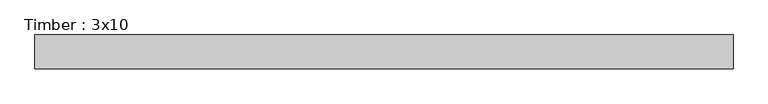
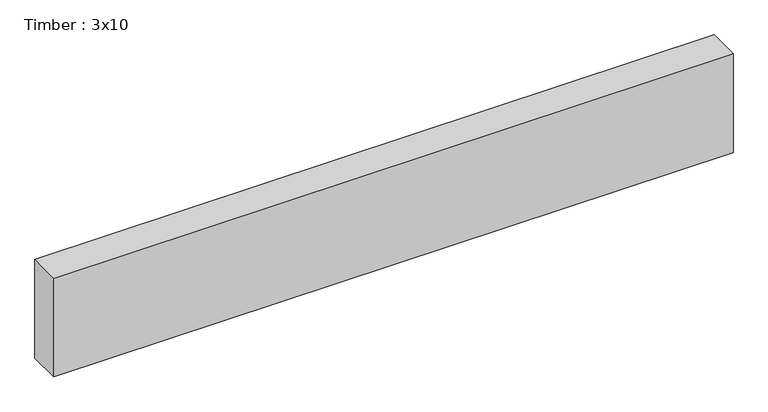
"""IFC4 building model written with IfcOpenShell, lengths in millimetres: beam geometry, Timber : 3x10."""

import ifcopenshell
import ifcopenshell.guid

model = None  # the IFC model being written
_history = None  # IfcOwnerHistory: only IFC2X3 demands one
_inside = {}  # id of a spatial element -> (the spatial element, [elements in it])
_under = {}  # id of a project, library or spatial element -> (it, [spatial elements below it])
_declared = {}  # id of a project -> (the project, [libraries it declares])
_typed = {}  # id of a type object -> (the type object, [elements of that type])
_made_of = {}  # id of a material, layer set ... -> (it, [elements and type objects made of it])


def new_model(schema):
    """Start an empty IFC model of exactly this schema.

    Asked for "IFC4X3", IfcOpenShell would pick the latest addendum, in which some entities
    have other attributes; the version numbers below select the first issue.
    IFC2X3 requires an IfcOwnerHistory on every rooted entity: one is made here for all.
    """
    global model, _history
    if schema == "IFC4X3":
        model = ifcopenshell.file(schema_version=(4, 3, 0, 0))
    else:
        model = ifcopenshell.file(schema=schema)
    _inside.clear()
    _under.clear()
    _declared.clear()
    _typed.clear()
    _made_of.clear()
    _history = None
    if model.schema == "IFC2X3":
        org = make("IfcOrganization", Name="unknown")
        user = make(
            "IfcPersonAndOrganization",
            ThePerson=make("IfcPerson", FamilyName="unknown"),
            TheOrganization=org,
        )
        app = make(
            "IfcApplication",
            ApplicationDeveloper=org,
            Version="unknown",
            ApplicationFullName="unknown",
            ApplicationIdentifier="unknown",
        )
        _history = make(
            "IfcOwnerHistory",
            OwningUser=user,
            OwningApplication=app,
            ChangeAction="ADDED",
            CreationDate=0,
        )
    return model


def make(cls, **values):
    """One entity of the class cls with the attributes given. An attribute that is None is left unset."""
    return model.create_entity(
        cls, **{name: value for name, value in values.items() if value is not None}
    )


def rooted(cls, **values):
    """An entity with a GlobalId (a new one), such as an element, a storey or a relation."""
    return make(cls, GlobalId=ifcopenshell.guid.new(), OwnerHistory=_history, **values)


def si_unit(unit_type, name, prefix=None):
    """IfcSIUnit, for example si_unit("LENGTHUNIT", "METRE", prefix="MILLI")."""
    return make("IfcSIUnit", UnitType=unit_type, Prefix=prefix, Name=name)


def assignment(units):
    """IfcUnitAssignment: the units of a project."""
    return None if units is None else make("IfcUnitAssignment", Units=units)


def point(xyz):
    """IfcCartesianPoint."""
    return None if xyz is None else make("IfcCartesianPoint", Coordinates=xyz)


def direction(xyz):
    """IfcDirection."""
    return None if xyz is None else make("IfcDirection", DirectionRatios=xyz)


def frame(location, z_axis=None, x_axis=None):
    """IfcAxis2Placement3D, a coordinate frame: its origin and axes. An axis left out is left unset."""
    return make(
        "IfcAxis2Placement3D",
        Location=point(location),
        Axis=direction(z_axis),
        RefDirection=direction(x_axis),
    )


def origin():
    """The frame at (0, 0, 0) with its axes left unset."""
    return frame((0.0, 0.0, 0.0))


def place(relative_to, where):
    """IfcLocalPlacement: puts the frame where relative to a parent placement (None: the world)."""
    return make(
        "IfcLocalPlacement", PlacementRelTo=relative_to, RelativePlacement=where
    )


def context(
    kind, dimensions, precision=None, world=None, true_north=None, identifier=None
):
    """IfcGeometricRepresentationContext, for example the 3D "Model" context."""
    return make(
        "IfcGeometricRepresentationContext",
        ContextIdentifier=identifier,
        ContextType=kind,
        CoordinateSpaceDimension=dimensions,
        Precision=precision,
        WorldCoordinateSystem=world,
        TrueNorth=true_north,
    )


def project(units=None, contexts=None):
    """IfcProject with its units and contexts."""
    return rooted(
        "IfcProject",
        Name="project",
        RepresentationContexts=contexts,
        UnitsInContext=assignment(units),
    )


def spatial(cls, under=None, at=None, **own):
    """A site, building, storey or space (cls), placed at a placement, below another one or the project."""
    s = rooted(cls, ObjectPlacement=at, **own)
    if under is not None:
        _under.setdefault(under.id(), (under, []))[1].append(s)
    return s


def polyline(points):
    """IfcPolyline through the points."""
    return make("IfcPolyline", Points=[point(p) for p in points])


def outline(outer, holes=None, kind="AREA"):
    """IfcArbitraryClosedProfileDef: a profile drawn as a closed curve; with holes, ...WithVoids."""
    if holes is None:
        return make("IfcArbitraryClosedProfileDef", ProfileType=kind, OuterCurve=outer)
    return make(
        "IfcArbitraryProfileDefWithVoids",
        ProfileType=kind,
        OuterCurve=outer,
        InnerCurves=holes,
    )


def extrude(swept, where, along, depth):
    """IfcExtrudedAreaSolid: the profile swept, set in the frame where, extruded along a direction by depth."""
    return make(
        "IfcExtrudedAreaSolid",
        SweptArea=swept,
        Position=where,
        ExtrudedDirection=direction(along),
        Depth=depth,
    )


def shape(context_of_items, identifier, shape_type, items):
    """IfcShapeRepresentation: the items that make up one representation, for example the "Body"."""
    return make(
        "IfcShapeRepresentation",
        ContextOfItems=context_of_items,
        RepresentationIdentifier=identifier,
        RepresentationType=shape_type,
        Items=items,
    )


def source(mapping_origin, context_of_items, identifier, shape_type, items):
    """IfcRepresentationMap: a shape defined once, which mapped items show again and again."""
    return make(
        "IfcRepresentationMap",
        MappingOrigin=mapping_origin,
        MappedRepresentation=shape(context_of_items, identifier, shape_type, items),
    )


def transform(
    local_origin,
    x_axis=None,
    y_axis=None,
    z_axis=None,
    scale=None,
    scale2=None,
    scale3=None,
    uniform=True,
):
    """IfcCartesianTransformationOperator3D, or its non-uniform kind. x_axis, y_axis, z_axis: its Axis1, 2, 3."""
    if uniform:
        return make(
            "IfcCartesianTransformationOperator3D",
            Axis1=direction(x_axis),
            Axis2=direction(y_axis),
            LocalOrigin=point(local_origin),
            Scale=scale,
            Axis3=direction(z_axis),
        )
    return make(
        "IfcCartesianTransformationOperator3DnonUniform",
        Axis1=direction(x_axis),
        Axis2=direction(y_axis),
        LocalOrigin=point(local_origin),
        Scale=scale,
        Axis3=direction(z_axis),
        Scale2=scale2,
        Scale3=scale3,
    )


def mapped(mapping_source, mapping_target):
    """IfcMappedItem: shows the shape of a source again, moved by a transform."""
    return make(
        "IfcMappedItem", MappingSource=mapping_source, MappingTarget=mapping_target
    )


def made_of(thing, what):
    """Note that an element or type object is made of a material, layer set ...; save() writes the relation."""
    if what is not None:
        _made_of.setdefault(what.id(), (what, []))[1].append(thing)
    return thing


def element(
    cls,
    number,
    at=None,
    inside=None,
    cuts=None,
    type_object=None,
    material=None,
    context=None,
    identifier="Body",
    shape_type=None,
    held_by="IfcProductDefinitionShape",
    body=None,
    shapes=None,
    **own,
):
    """One element of the class cls, such as IfcWall. Its Tag is "e" and its number.

    at: its placement. inside: the storey or other place that contains it. cuts: it is an
    opening in that element (IfcRelVoidsElement). A single representation is given by context,
    identifier, shape_type and body (its items); several are given by shapes. held_by: the class
    of the entity that holds the representations. save() writes the other relations.
    """
    e = rooted(cls, Tag="e%d" % number, ObjectPlacement=at, **own)
    if body is not None:
        shapes = [shape(context, identifier, shape_type, body)]
    if shapes is not None:
        e.Representation = make(held_by, Representations=shapes)
    if inside is not None:
        _inside.setdefault(inside.id(), (inside, []))[1].append(e)
    if cuts is not None:
        rooted(
            "IfcRelVoidsElement", RelatingBuildingElement=cuts, RelatedOpeningElement=e
        )
    if type_object is not None:
        _typed.setdefault(type_object.id(), (type_object, []))[1].append(e)
    return made_of(e, material)


def aggregate(whole, parts):
    """IfcRelAggregates: a whole, such as a stair, and the parts it consists of."""
    return rooted("IfcRelAggregates", RelatingObject=whole, RelatedObjects=parts)


def save(model, path):
    """Write the relations noted so far, then the file.

    IfcRelAggregates (storeys below a building ...), IfcRelContainedInSpatialStructure (elements
    in a storey), IfcRelDefinesByType, IfcRelAssociatesMaterial and IfcRelDeclares: one each for
    every whole, place, type object, material and project.
    """
    for whole, parts in _under.values():
        aggregate(whole, parts)
    for where, things in _inside.values():
        rooted(
            "IfcRelContainedInSpatialStructure",
            RelatedElements=things,
            RelatingStructure=where,
        )
    for kind, things in _typed.values():
        rooted("IfcRelDefinesByType", RelatedObjects=things, RelatingType=kind)
    for what, things in _made_of.values():
        rooted("IfcRelAssociatesMaterial", RelatedObjects=things, RelatingMaterial=what)
    for by, libraries in _declared.values():
        rooted("IfcRelDeclares", RelatingContext=by, RelatedDefinitions=libraries)
    model.write(path)


def timber_3x10_88a0bdfd(model_context):
    return source(origin(), model_context, "Body", "SweptSolid", [
        extrude(outline(polyline([(785.1325751, 38.1), (785.1325751, -38.1), (-785.1325751, -38.1), (-785.1325751, 38.1), (785.1325751, 38.1)])), frame((0.0, 0.0, -120.65), z_axis=(0.0, 0.0, 1.0), x_axis=(1.0, 0.0, 0.0)), (0.0, 0.0, 1.0), 241.3),
    ])


if __name__ == "__main__":
    model = new_model("IFC4")
    model_context = context("Model", 3, world=origin())
    ifc_project = project(units=[si_unit("LENGTHUNIT", "METRE", prefix="MILLI")], contexts=[model_context])
    site = spatial("IfcSite", under=ifc_project)
    building = spatial("IfcBuilding", under=site)
    placement = place(None, origin())
    timber_3x10_shape = timber_3x10_88a0bdfd(model_context)
    element("IfcBeam", 1, ObjectType="Timber : 3x10", at=placement, inside=building, context=model_context, shape_type="MappedRepresentation", body=[
        mapped(timber_3x10_shape, transform((0.0, 0.0, 0.0), x_axis=(1.0, 0.0, 0.0), y_axis=(0.0, 1.0, 0.0), z_axis=(0.0, 0.0, 1.0))),
    ])
    save(model, "model.ifc")

# Revit data of these elements
# Type "Timber : 3x10"
#   Assembly Code = "B10"
#   A = 0.362847 SF
#   Length [instance default] = 5' - 0"
#   b = 0' - 3"
#   d = 0' - 9 1/2"
#   Structural Material [instance default] = Softwood, Lumber
# Element 1 (IfcBeam, "Timber : 3x10")
#   Materials on its faces: "Softwood, Lumber"
# Materials
#   "Softwood, Lumber": class "Wood", colour RGB 144 113 62, transparency 0, Description = "Pinus Echinata", Cost = 0
